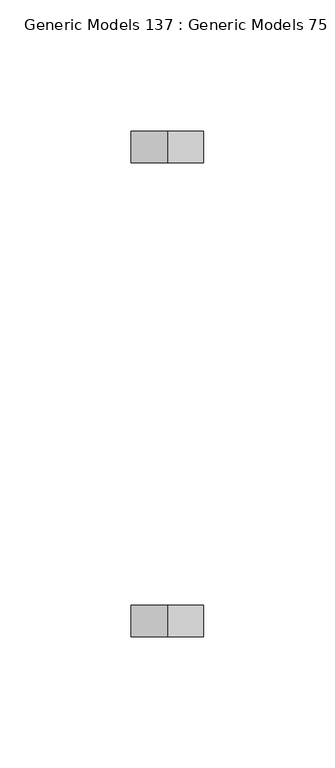
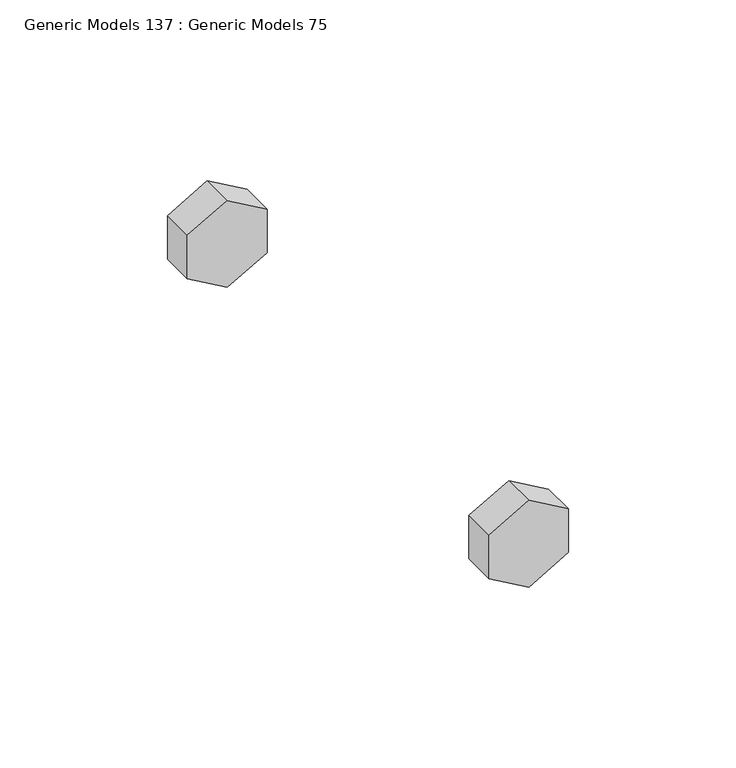
"""IFC4 building model written with IfcOpenShell, lengths in millimetres: proxy geometry, Generic Models 137 : Generic Models 75."""

from ifc_helpers import new_model, si_unit, frame, origin, place, context, project, spatial, polyline, outline, extrude, source, transform, mapped, element, save


def generic_models_137_generic_models_75_a24f89dc(model_context):
    return source(origin(), model_context, "Body", "SweptSolid", [
        extrude(outline(polyline([(269222.3462802, 31974.4067029), (269206.5097067, 31974.4067029), (269198.59142, 31988.1215778), (269206.5097067, 32001.8364528), (269222.3462802, 32001.8364528), (269230.264567, 31988.1215778), (269222.3462802, 31974.4067029)])), frame((0.0, 36491.5582942, 0.0), z_axis=(0.0, 1.0, 0.0), x_axis=(0.0, 0.0, 1.0)), (0.0, 0.0, 1.0), 11.90625),
        extrude(outline(polyline([(269222.3462802, 31974.4067029), (269206.5097067, 31974.4067029), (269198.59142, 31988.1215778), (269206.5097067, 32001.8364528), (269222.3462802, 32001.8364528), (269230.264567, 31988.1215778), (269222.3462802, 31974.4067029)])), frame((0.0, 36311.3770442, 0.0), z_axis=(0.0, 1.0, 0.0), x_axis=(0.0, 0.0, 1.0)), (0.0, 0.0, 1.0), 11.90625),
    ])


if __name__ == "__main__":
    model = new_model("IFC4")
    model_context = context("Model", 3, world=origin())
    ifc_project = project(units=[si_unit("LENGTHUNIT", "METRE", prefix="MILLI")], contexts=[model_context])
    site = spatial("IfcSite", under=ifc_project)
    building = spatial("IfcBuilding", under=site)
    placement = place(None, origin())
    generic_models_137_generic_models_75_shape = generic_models_137_generic_models_75_a24f89dc(model_context)
    element("IfcBuildingElementProxy", 1, Name="Generic Models 137 : Generic Models 75", ObjectType="Generic Models 137 : Generic Models 75", at=placement, inside=building, context=model_context, shape_type="MappedRepresentation", body=[
        mapped(generic_models_137_generic_models_75_shape, transform((0.0, 0.0, 0.0), x_axis=(1.0, 0.0, 0.0), y_axis=(0.0, 1.0, 0.0), z_axis=(0.0, 0.0, 1.0))),
    ])
    save(model, "model.ifc")

# Revit data of these elements
# Element 1 (IfcBuildingElementProxy, "Generic Models 137 : Generic Models 75")
#   Materials on its faces: "3/4\" GALV. THRU BOLTS"
# Materials
#   "3/4\" GALV. THRU BOLTS": class "Generic", colour RGB 105 69 171, transparency 0, Cost = 0
